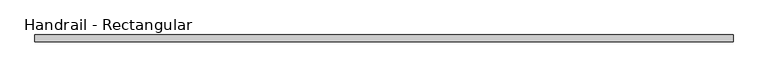
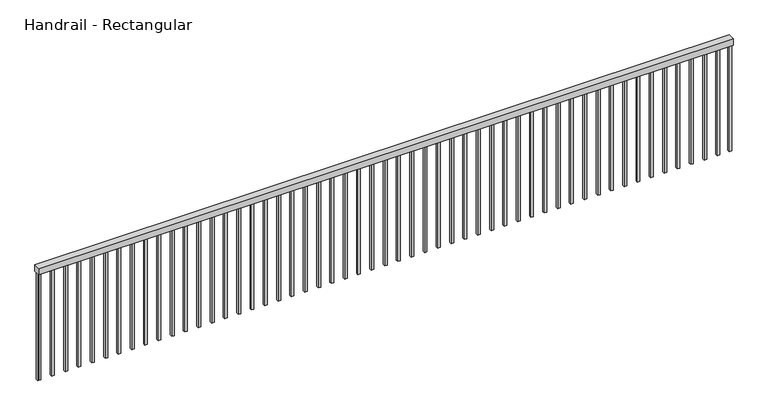
"""IFC4 building model written with IfcOpenShell, lengths in millimetres: railing geometry, Handrail - Rectangular."""

from ifc_helpers import new_model, si_unit, frame, origin, place, context, project, spatial, polyline, outline, extrude, source, transform, mapped, element, save


def handrail_rectangular_538153ec(model_context):
    return source(origin(), model_context, "Body", "SweptSolid", [
        extrude(outline(polyline([(2034.7788909, 4871.6507146), (2034.7788909, 4820.8507146), (-3265.2211091, 4820.8507146), (-3265.2211091, 4871.6507146), (2034.7788909, 4871.6507146)])), frame((0.0, 0.0, 6654.4), z_axis=(0.0, 0.0, 1.0), x_axis=(1.0, 0.0, 0.0)), (0.0, 0.0, 1.0), 50.8),
        extrude(outline(polyline([(-3238.8961091, 4855.7757146), (-3238.8961091, 4836.7257146), (-3257.9461091, 4836.7257146), (-3257.9461091, 4855.7757146), (-3238.8961091, 4855.7757146)])), frame((0.0, 0.0, 5790.8), z_axis=(0.0, 0.0, 1.0), x_axis=(1.0, 0.0, 0.0)), (0.0, 0.0, 1.0), 863.6),
        extrude(outline(polyline([(-3137.2961091, 4855.7757146), (-3137.2961091, 4836.7257146), (-3156.3461091, 4836.7257146), (-3156.3461091, 4855.7757146), (-3137.2961091, 4855.7757146)])), frame((0.0, 0.0, 5790.8), z_axis=(0.0, 0.0, 1.0), x_axis=(1.0, 0.0, 0.0)), (0.0, 0.0, 1.0), 863.6),
        extrude(outline(polyline([(-3035.6961091, 4855.7757146), (-3035.6961091, 4836.7257146), (-3054.7461091, 4836.7257146), (-3054.7461091, 4855.7757146), (-3035.6961091, 4855.7757146)])), frame((0.0, 0.0, 5790.8), z_axis=(0.0, 0.0, 1.0), x_axis=(1.0, 0.0, 0.0)), (0.0, 0.0, 1.0), 863.6),
        extrude(outline(polyline([(-2934.0961091, 4855.7757146), (-2934.0961091, 4836.7257146), (-2953.1461091, 4836.7257146), (-2953.1461091, 4855.7757146), (-2934.0961091, 4855.7757146)])), frame((0.0, 0.0, 5790.8), z_axis=(0.0, 0.0, 1.0), x_axis=(1.0, 0.0, 0.0)), (0.0, 0.0, 1.0), 863.6),
        extrude(outline(polyline([(-2832.4961091, 4855.7757146), (-2832.4961091, 4836.7257146), (-2851.5461091, 4836.7257146), (-2851.5461091, 4855.7757146), (-2832.4961091, 4855.7757146)])), frame((0.0, 0.0, 5790.8), z_axis=(0.0, 0.0, 1.0), x_axis=(1.0, 0.0, 0.0)), (0.0, 0.0, 1.0), 863.6),
        extrude(outline(polyline([(-2730.8961091, 4855.7757146), (-2730.8961091, 4836.7257146), (-2749.9461091, 4836.7257146), (-2749.9461091, 4855.7757146), (-2730.8961091, 4855.7757146)])), frame((0.0, 0.0, 5790.8), z_axis=(0.0, 0.0, 1.0), x_axis=(1.0, 0.0, 0.0)), (0.0, 0.0, 1.0), 863.6),
        extrude(outline(polyline([(-2629.2961091, 4855.7757146), (-2629.2961091, 4836.7257146), (-2648.3461091, 4836.7257146), (-2648.3461091, 4855.7757146), (-2629.2961091, 4855.7757146)])), frame((0.0, 0.0, 5790.8), z_axis=(0.0, 0.0, 1.0), x_axis=(1.0, 0.0, 0.0)), (0.0, 0.0, 1.0), 863.6),
        extrude(outline(polyline([(-2527.6961091, 4855.7757146), (-2527.6961091, 4836.7257146), (-2546.7461091, 4836.7257146), (-2546.7461091, 4855.7757146), (-2527.6961091, 4855.7757146)])), frame((0.0, 0.0, 5790.8), z_axis=(0.0, 0.0, 1.0), x_axis=(1.0, 0.0, 0.0)), (0.0, 0.0, 1.0), 863.6),
        extrude(outline(polyline([(-2426.0961091, 4855.7757146), (-2426.0961091, 4836.7257146), (-2445.1461091, 4836.7257146), (-2445.1461091, 4855.7757146), (-2426.0961091, 4855.7757146)])), frame((0.0, 0.0, 5790.8), z_axis=(0.0, 0.0, 1.0), x_axis=(1.0, 0.0, 0.0)), (0.0, 0.0, 1.0), 863.6),
        extrude(outline(polyline([(-2324.4961091, 4855.7757146), (-2324.4961091, 4836.7257146), (-2343.5461091, 4836.7257146), (-2343.5461091, 4855.7757146), (-2324.4961091, 4855.7757146)])), frame((0.0, 0.0, 5790.8), z_axis=(0.0, 0.0, 1.0), x_axis=(1.0, 0.0, 0.0)), (0.0, 0.0, 1.0), 863.6),
        extrude(outline(polyline([(-2222.8961091, 4855.7757146), (-2222.8961091, 4836.7257146), (-2241.9461091, 4836.7257146), (-2241.9461091, 4855.7757146), (-2222.8961091, 4855.7757146)])), frame((0.0, 0.0, 5790.8), z_axis=(0.0, 0.0, 1.0), x_axis=(1.0, 0.0, 0.0)), (0.0, 0.0, 1.0), 863.6),
        extrude(outline(polyline([(-2121.2961091, 4855.7757146), (-2121.2961091, 4836.7257146), (-2140.3461091, 4836.7257146), (-2140.3461091, 4855.7757146), (-2121.2961091, 4855.7757146)])), frame((0.0, 0.0, 5790.8), z_axis=(0.0, 0.0, 1.0), x_axis=(1.0, 0.0, 0.0)), (0.0, 0.0, 1.0), 863.6),
        extrude(outline(polyline([(-2019.6961091, 4855.7757146), (-2019.6961091, 4836.7257146), (-2038.7461091, 4836.7257146), (-2038.7461091, 4855.7757146), (-2019.6961091, 4855.7757146)])), frame((0.0, 0.0, 5790.8), z_axis=(0.0, 0.0, 1.0), x_axis=(1.0, 0.0, 0.0)), (0.0, 0.0, 1.0), 863.6),
        extrude(outline(polyline([(-1918.0961091, 4855.7757146), (-1918.0961091, 4836.7257146), (-1937.1461091, 4836.7257146), (-1937.1461091, 4855.7757146), (-1918.0961091, 4855.7757146)])), frame((0.0, 0.0, 5790.8), z_axis=(0.0, 0.0, 1.0), x_axis=(1.0, 0.0, 0.0)), (0.0, 0.0, 1.0), 863.6),
        extrude(outline(polyline([(-1816.4961091, 4855.7757146), (-1816.4961091, 4836.7257146), (-1835.5461091, 4836.7257146), (-1835.5461091, 4855.7757146), (-1816.4961091, 4855.7757146)])), frame((0.0, 0.0, 5790.8), z_axis=(0.0, 0.0, 1.0), x_axis=(1.0, 0.0, 0.0)), (0.0, 0.0, 1.0), 863.6),
        extrude(outline(polyline([(-1714.8961091, 4855.7757146), (-1714.8961091, 4836.7257146), (-1733.9461091, 4836.7257146), (-1733.9461091, 4855.7757146), (-1714.8961091, 4855.7757146)])), frame((0.0, 0.0, 5790.8), z_axis=(0.0, 0.0, 1.0), x_axis=(1.0, 0.0, 0.0)), (0.0, 0.0, 1.0), 863.6),
        extrude(outline(polyline([(-1613.2961091, 4855.7757146), (-1613.2961091, 4836.7257146), (-1632.3461091, 4836.7257146), (-1632.3461091, 4855.7757146), (-1613.2961091, 4855.7757146)])), frame((0.0, 0.0, 5790.8), z_axis=(0.0, 0.0, 1.0), x_axis=(1.0, 0.0, 0.0)), (0.0, 0.0, 1.0), 863.6),
        extrude(outline(polyline([(-1511.6961091, 4855.7757146), (-1511.6961091, 4836.7257146), (-1530.7461091, 4836.7257146), (-1530.7461091, 4855.7757146), (-1511.6961091, 4855.7757146)])), frame((0.0, 0.0, 5790.8), z_axis=(0.0, 0.0, 1.0), x_axis=(1.0, 0.0, 0.0)), (0.0, 0.0, 1.0), 863.6),
        extrude(outline(polyline([(-1410.0961091, 4855.7757146), (-1410.0961091, 4836.7257146), (-1429.1461091, 4836.7257146), (-1429.1461091, 4855.7757146), (-1410.0961091, 4855.7757146)])), frame((0.0, 0.0, 5790.8), z_axis=(0.0, 0.0, 1.0), x_axis=(1.0, 0.0, 0.0)), (0.0, 0.0, 1.0), 863.6),
        extrude(outline(polyline([(-1308.4961091, 4855.7757146), (-1308.4961091, 4836.7257146), (-1327.5461091, 4836.7257146), (-1327.5461091, 4855.7757146), (-1308.4961091, 4855.7757146)])), frame((0.0, 0.0, 5790.8), z_axis=(0.0, 0.0, 1.0), x_axis=(1.0, 0.0, 0.0)), (0.0, 0.0, 1.0), 863.6),
        extrude(outline(polyline([(-1206.8961091, 4855.7757146), (-1206.8961091, 4836.7257146), (-1225.9461091, 4836.7257146), (-1225.9461091, 4855.7757146), (-1206.8961091, 4855.7757146)])), frame((0.0, 0.0, 5790.8), z_axis=(0.0, 0.0, 1.0), x_axis=(1.0, 0.0, 0.0)), (0.0, 0.0, 1.0), 863.6),
        extrude(outline(polyline([(-1105.2961091, 4855.7757146), (-1105.2961091, 4836.7257146), (-1124.3461091, 4836.7257146), (-1124.3461091, 4855.7757146), (-1105.2961091, 4855.7757146)])), frame((0.0, 0.0, 5790.8), z_axis=(0.0, 0.0, 1.0), x_axis=(1.0, 0.0, 0.0)), (0.0, 0.0, 1.0), 863.6),
        extrude(outline(polyline([(-1003.6961091, 4855.7757146), (-1003.6961091, 4836.7257146), (-1022.7461091, 4836.7257146), (-1022.7461091, 4855.7757146), (-1003.6961091, 4855.7757146)])), frame((0.0, 0.0, 5790.8), z_axis=(0.0, 0.0, 1.0), x_axis=(1.0, 0.0, 0.0)), (0.0, 0.0, 1.0), 863.6),
        extrude(outline(polyline([(-902.0961091, 4855.7757146), (-902.0961091, 4836.7257146), (-921.1461091, 4836.7257146), (-921.1461091, 4855.7757146), (-902.0961091, 4855.7757146)])), frame((0.0, 0.0, 5790.8), z_axis=(0.0, 0.0, 1.0), x_axis=(1.0, 0.0, 0.0)), (0.0, 0.0, 1.0), 863.6),
        extrude(outline(polyline([(-800.4961091, 4855.7757146), (-800.4961091, 4836.7257146), (-819.5461091, 4836.7257146), (-819.5461091, 4855.7757146), (-800.4961091, 4855.7757146)])), frame((0.0, 0.0, 5790.8), z_axis=(0.0, 0.0, 1.0), x_axis=(1.0, 0.0, 0.0)), (0.0, 0.0, 1.0), 863.6),
        extrude(outline(polyline([(-698.8961091, 4855.7757146), (-698.8961091, 4836.7257146), (-717.9461091, 4836.7257146), (-717.9461091, 4855.7757146), (-698.8961091, 4855.7757146)])), frame((0.0, 0.0, 5790.8), z_axis=(0.0, 0.0, 1.0), x_axis=(1.0, 0.0, 0.0)), (0.0, 0.0, 1.0), 863.6),
        extrude(outline(polyline([(-597.2961091, 4855.7757146), (-597.2961091, 4836.7257146), (-616.3461091, 4836.7257146), (-616.3461091, 4855.7757146), (-597.2961091, 4855.7757146)])), frame((0.0, 0.0, 5790.8), z_axis=(0.0, 0.0, 1.0), x_axis=(1.0, 0.0, 0.0)), (0.0, 0.0, 1.0), 863.6),
        extrude(outline(polyline([(-495.6961091, 4855.7757146), (-495.6961091, 4836.7257146), (-514.7461091, 4836.7257146), (-514.7461091, 4855.7757146), (-495.6961091, 4855.7757146)])), frame((0.0, 0.0, 5790.8), z_axis=(0.0, 0.0, 1.0), x_axis=(1.0, 0.0, 0.0)), (0.0, 0.0, 1.0), 863.6),
        extrude(outline(polyline([(-394.0961091, 4855.7757146), (-394.0961091, 4836.7257146), (-413.1461091, 4836.7257146), (-413.1461091, 4855.7757146), (-394.0961091, 4855.7757146)])), frame((0.0, 0.0, 5790.8), z_axis=(0.0, 0.0, 1.0), x_axis=(1.0, 0.0, 0.0)), (0.0, 0.0, 1.0), 863.6),
        extrude(outline(polyline([(-292.4961091, 4855.7757146), (-292.4961091, 4836.7257146), (-311.5461091, 4836.7257146), (-311.5461091, 4855.7757146), (-292.4961091, 4855.7757146)])), frame((0.0, 0.0, 5790.8), z_axis=(0.0, 0.0, 1.0), x_axis=(1.0, 0.0, 0.0)), (0.0, 0.0, 1.0), 863.6),
        extrude(outline(polyline([(-190.8961091, 4855.7757146), (-190.8961091, 4836.7257146), (-209.9461091, 4836.7257146), (-209.9461091, 4855.7757146), (-190.8961091, 4855.7757146)])), frame((0.0, 0.0, 5790.8), z_axis=(0.0, 0.0, 1.0), x_axis=(1.0, 0.0, 0.0)), (0.0, 0.0, 1.0), 863.6),
        extrude(outline(polyline([(-89.2961091, 4855.7757146), (-89.2961091, 4836.7257146), (-108.3461091, 4836.7257146), (-108.3461091, 4855.7757146), (-89.2961091, 4855.7757146)])), frame((0.0, 0.0, 5790.8), z_axis=(0.0, 0.0, 1.0), x_axis=(1.0, 0.0, 0.0)), (0.0, 0.0, 1.0), 863.6),
        extrude(outline(polyline([(12.3038909, 4855.7757146), (12.3038909, 4836.7257146), (-6.7461091, 4836.7257146), (-6.7461091, 4855.7757146), (12.3038909, 4855.7757146)])), frame((0.0, 0.0, 5790.8), z_axis=(0.0, 0.0, 1.0), x_axis=(1.0, 0.0, 0.0)), (0.0, 0.0, 1.0), 863.6),
        extrude(outline(polyline([(113.9038909, 4855.7757146), (113.9038909, 4836.7257146), (94.8538909, 4836.7257146), (94.8538909, 4855.7757146), (113.9038909, 4855.7757146)])), frame((0.0, 0.0, 5790.8), z_axis=(0.0, 0.0, 1.0), x_axis=(1.0, 0.0, 0.0)), (0.0, 0.0, 1.0), 863.6),
        extrude(outline(polyline([(215.5038909, 4855.7757146), (215.5038909, 4836.7257146), (196.4538909, 4836.7257146), (196.4538909, 4855.7757146), (215.5038909, 4855.7757146)])), frame((0.0, 0.0, 5790.8), z_axis=(0.0, 0.0, 1.0), x_axis=(1.0, 0.0, 0.0)), (0.0, 0.0, 1.0), 863.6),
        extrude(outline(polyline([(317.1038909, 4855.7757146), (317.1038909, 4836.7257146), (298.0538909, 4836.7257146), (298.0538909, 4855.7757146), (317.1038909, 4855.7757146)])), frame((0.0, 0.0, 5790.8), z_axis=(0.0, 0.0, 1.0), x_axis=(1.0, 0.0, 0.0)), (0.0, 0.0, 1.0), 863.6),
        extrude(outline(polyline([(418.7038909, 4855.7757146), (418.7038909, 4836.7257146), (399.6538909, 4836.7257146), (399.6538909, 4855.7757146), (418.7038909, 4855.7757146)])), frame((0.0, 0.0, 5790.8), z_axis=(0.0, 0.0, 1.0), x_axis=(1.0, 0.0, 0.0)), (0.0, 0.0, 1.0), 863.6),
        extrude(outline(polyline([(520.3038909, 4855.7757146), (520.3038909, 4836.7257146), (501.2538909, 4836.7257146), (501.2538909, 4855.7757146), (520.3038909, 4855.7757146)])), frame((0.0, 0.0, 5790.8), z_axis=(0.0, 0.0, 1.0), x_axis=(1.0, 0.0, 0.0)), (0.0, 0.0, 1.0), 863.6),
        extrude(outline(polyline([(621.9038909, 4855.7757146), (621.9038909, 4836.7257146), (602.8538909, 4836.7257146), (602.8538909, 4855.7757146), (621.9038909, 4855.7757146)])), frame((0.0, 0.0, 5790.8), z_axis=(0.0, 0.0, 1.0), x_axis=(1.0, 0.0, 0.0)), (0.0, 0.0, 1.0), 863.6),
        extrude(outline(polyline([(723.5038909, 4855.7757146), (723.5038909, 4836.7257146), (704.4538909, 4836.7257146), (704.4538909, 4855.7757146), (723.5038909, 4855.7757146)])), frame((0.0, 0.0, 5790.8), z_axis=(0.0, 0.0, 1.0), x_axis=(1.0, 0.0, 0.0)), (0.0, 0.0, 1.0), 863.6),
        extrude(outline(polyline([(825.1038909, 4855.7757146), (825.1038909, 4836.7257146), (806.0538909, 4836.7257146), (806.0538909, 4855.7757146), (825.1038909, 4855.7757146)])), frame((0.0, 0.0, 5790.8), z_axis=(0.0, 0.0, 1.0), x_axis=(1.0, 0.0, 0.0)), (0.0, 0.0, 1.0), 863.6),
        extrude(outline(polyline([(926.7038909, 4855.7757146), (926.7038909, 4836.7257146), (907.6538909, 4836.7257146), (907.6538909, 4855.7757146), (926.7038909, 4855.7757146)])), frame((0.0, 0.0, 5790.8), z_axis=(0.0, 0.0, 1.0), x_axis=(1.0, 0.0, 0.0)), (0.0, 0.0, 1.0), 863.6),
        extrude(outline(polyline([(1028.3038909, 4855.7757146), (1028.3038909, 4836.7257146), (1009.2538909, 4836.7257146), (1009.2538909, 4855.7757146), (1028.3038909, 4855.7757146)])), frame((0.0, 0.0, 5790.8), z_axis=(0.0, 0.0, 1.0), x_axis=(1.0, 0.0, 0.0)), (0.0, 0.0, 1.0), 863.6),
        extrude(outline(polyline([(1129.9038909, 4855.7757146), (1129.9038909, 4836.7257146), (1110.8538909, 4836.7257146), (1110.8538909, 4855.7757146), (1129.9038909, 4855.7757146)])), frame((0.0, 0.0, 5790.8), z_axis=(0.0, 0.0, 1.0), x_axis=(1.0, 0.0, 0.0)), (0.0, 0.0, 1.0), 863.6),
        extrude(outline(polyline([(1231.5038909, 4855.7757146), (1231.5038909, 4836.7257146), (1212.4538909, 4836.7257146), (1212.4538909, 4855.7757146), (1231.5038909, 4855.7757146)])), frame((0.0, 0.0, 5790.8), z_axis=(0.0, 0.0, 1.0), x_axis=(1.0, 0.0, 0.0)), (0.0, 0.0, 1.0), 863.6),
        extrude(outline(polyline([(1333.1038909, 4855.7757146), (1333.1038909, 4836.7257146), (1314.0538909, 4836.7257146), (1314.0538909, 4855.7757146), (1333.1038909, 4855.7757146)])), frame((0.0, 0.0, 5790.8), z_axis=(0.0, 0.0, 1.0), x_axis=(1.0, 0.0, 0.0)), (0.0, 0.0, 1.0), 863.6),
        extrude(outline(polyline([(1434.7038909, 4855.7757146), (1434.7038909, 4836.7257146), (1415.6538909, 4836.7257146), (1415.6538909, 4855.7757146), (1434.7038909, 4855.7757146)])), frame((0.0, 0.0, 5790.8), z_axis=(0.0, 0.0, 1.0), x_axis=(1.0, 0.0, 0.0)), (0.0, 0.0, 1.0), 863.6),
        extrude(outline(polyline([(1536.3038909, 4855.7757146), (1536.3038909, 4836.7257146), (1517.2538909, 4836.7257146), (1517.2538909, 4855.7757146), (1536.3038909, 4855.7757146)])), frame((0.0, 0.0, 5790.8), z_axis=(0.0, 0.0, 1.0), x_axis=(1.0, 0.0, 0.0)), (0.0, 0.0, 1.0), 863.6),
        extrude(outline(polyline([(1637.9038909, 4855.7757146), (1637.9038909, 4836.7257146), (1618.8538909, 4836.7257146), (1618.8538909, 4855.7757146), (1637.9038909, 4855.7757146)])), frame((0.0, 0.0, 5790.8), z_axis=(0.0, 0.0, 1.0), x_axis=(1.0, 0.0, 0.0)), (0.0, 0.0, 1.0), 863.6),
        extrude(outline(polyline([(1739.5038909, 4855.7757146), (1739.5038909, 4836.7257146), (1720.4538909, 4836.7257146), (1720.4538909, 4855.7757146), (1739.5038909, 4855.7757146)])), frame((0.0, 0.0, 5790.8), z_axis=(0.0, 0.0, 1.0), x_axis=(1.0, 0.0, 0.0)), (0.0, 0.0, 1.0), 863.6),
        extrude(outline(polyline([(1841.1038909, 4855.7757146), (1841.1038909, 4836.7257146), (1822.0538909, 4836.7257146), (1822.0538909, 4855.7757146), (1841.1038909, 4855.7757146)])), frame((0.0, 0.0, 5790.8), z_axis=(0.0, 0.0, 1.0), x_axis=(1.0, 0.0, 0.0)), (0.0, 0.0, 1.0), 863.6),
        extrude(outline(polyline([(1942.7038909, 4855.7757146), (1942.7038909, 4836.7257146), (1923.6538909, 4836.7257146), (1923.6538909, 4855.7757146), (1942.7038909, 4855.7757146)])), frame((0.0, 0.0, 5790.8), z_axis=(0.0, 0.0, 1.0), x_axis=(1.0, 0.0, 0.0)), (0.0, 0.0, 1.0), 863.6),
        extrude(outline(polyline([(-3246.1711091, 4855.7757146), (-3246.1711091, 4836.7257146), (-3265.2211091, 4836.7257146), (-3265.2211091, 4855.7757146), (-3246.1711091, 4855.7757146)])), frame((0.0, 0.0, 5790.8), z_axis=(0.0, 0.0, 1.0), x_axis=(1.0, 0.0, 0.0)), (0.0, 0.0, 1.0), 863.6),
        extrude(outline(polyline([(2034.7788909, 4855.7757146), (2034.7788909, 4836.7257146), (2015.7288909, 4836.7257146), (2015.7288909, 4855.7757146), (2034.7788909, 4855.7757146)])), frame((0.0, 0.0, 5790.8), z_axis=(0.0, 0.0, 1.0), x_axis=(1.0, 0.0, 0.0)), (0.0, 0.0, 1.0), 863.6),
    ])


if __name__ == "__main__":
    model = new_model("IFC4")
    model_context = context("Model", 3, world=origin())
    ifc_project = project(units=[si_unit("LENGTHUNIT", "METRE", prefix="MILLI")], contexts=[model_context])
    site = spatial("IfcSite", under=ifc_project)
    building = spatial("IfcBuilding", under=site)
    placement = place(None, origin())
    handrail_rectangular_shape = handrail_rectangular_538153ec(model_context)
    element("IfcRailing", 1, ObjectType="Handrail - Rectangular", at=placement, inside=building, context=model_context, shape_type="MappedRepresentation", body=[
        mapped(handrail_rectangular_shape, transform((0.0, 0.0, 0.0), x_axis=(1.0, 0.0, 0.0), y_axis=(0.0, 1.0, 0.0), z_axis=(0.0, 0.0, 1.0))),
    ])
    save(model, "model.ifc")
